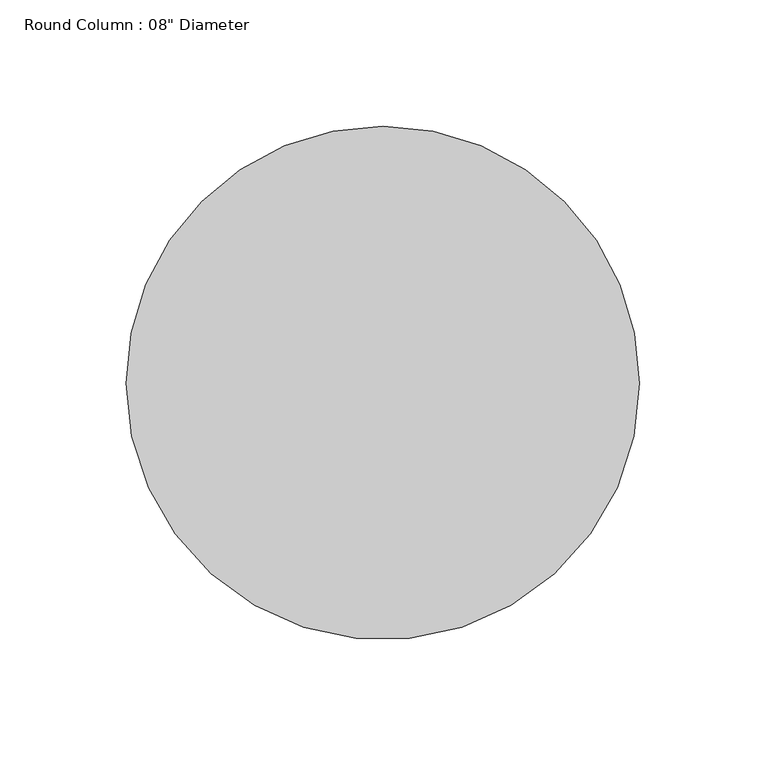
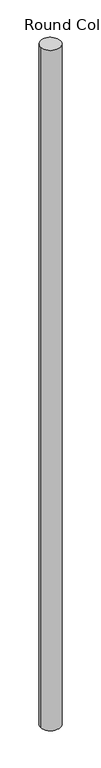
"""IFC4 building model written with IfcOpenShell, lengths in millimetres: column geometry."""

import ifcopenshell
import ifcopenshell.guid

model = None  # the IFC model being written
_history = None  # IfcOwnerHistory: only IFC2X3 demands one
_inside = {}  # id of a spatial element -> (the spatial element, [elements in it])
_under = {}  # id of a project, library or spatial element -> (it, [spatial elements below it])
_declared = {}  # id of a project -> (the project, [libraries it declares])
_typed = {}  # id of a type object -> (the type object, [elements of that type])
_made_of = {}  # id of a material, layer set ... -> (it, [elements and type objects made of it])


def new_model(schema):
    """Start an empty IFC model of exactly this schema.

    Asked for "IFC4X3", IfcOpenShell would pick the latest addendum, in which some entities
    have other attributes; the version numbers below select the first issue.
    IFC2X3 requires an IfcOwnerHistory on every rooted entity: one is made here for all.
    """
    global model, _history
    if schema == "IFC4X3":
        model = ifcopenshell.file(schema_version=(4, 3, 0, 0))
    else:
        model = ifcopenshell.file(schema=schema)
    _inside.clear()
    _under.clear()
    _declared.clear()
    _typed.clear()
    _made_of.clear()
    _history = None
    if model.schema == "IFC2X3":
        org = make("IfcOrganization", Name="unknown")
        user = make(
            "IfcPersonAndOrganization",
            ThePerson=make("IfcPerson", FamilyName="unknown"),
            TheOrganization=org,
        )
        app = make(
            "IfcApplication",
            ApplicationDeveloper=org,
            Version="unknown",
            ApplicationFullName="unknown",
            ApplicationIdentifier="unknown",
        )
        _history = make(
            "IfcOwnerHistory",
            OwningUser=user,
            OwningApplication=app,
            ChangeAction="ADDED",
            CreationDate=0,
        )
    return model


def make(cls, **values):
    """One entity of the class cls with the attributes given. An attribute that is None is left unset."""
    return model.create_entity(
        cls, **{name: value for name, value in values.items() if value is not None}
    )


def rooted(cls, **values):
    """An entity with a GlobalId (a new one), such as an element, a storey or a relation."""
    return make(cls, GlobalId=ifcopenshell.guid.new(), OwnerHistory=_history, **values)


def si_unit(unit_type, name, prefix=None):
    """IfcSIUnit, for example si_unit("LENGTHUNIT", "METRE", prefix="MILLI")."""
    return make("IfcSIUnit", UnitType=unit_type, Prefix=prefix, Name=name)


def assignment(units):
    """IfcUnitAssignment: the units of a project."""
    return None if units is None else make("IfcUnitAssignment", Units=units)


def point(xyz):
    """IfcCartesianPoint."""
    return None if xyz is None else make("IfcCartesianPoint", Coordinates=xyz)


def direction(xyz):
    """IfcDirection."""
    return None if xyz is None else make("IfcDirection", DirectionRatios=xyz)


def frame(location, z_axis=None, x_axis=None):
    """IfcAxis2Placement3D, a coordinate frame: its origin and axes. An axis left out is left unset."""
    return make(
        "IfcAxis2Placement3D",
        Location=point(location),
        Axis=direction(z_axis),
        RefDirection=direction(x_axis),
    )


def frame_2d(location, x_axis=None):
    """IfcAxis2Placement2D, a coordinate frame in the plane: its origin and x axis."""
    return make(
        "IfcAxis2Placement2D", Location=point(location), RefDirection=direction(x_axis)
    )


def origin():
    """The frame at (0, 0, 0) with its axes left unset."""
    return frame((0.0, 0.0, 0.0))


def origin_with_axes():
    """The frame at (0, 0, 0) with the z axis (0, 0, 1) and the x axis (1, 0, 0) written out."""
    return frame((0.0, 0.0, 0.0), z_axis=(0.0, 0.0, 1.0), x_axis=(1.0, 0.0, 0.0))


def origin_2d():
    """The frame at (0, 0) in the plane with its x axis left unset."""
    return frame_2d((0.0, 0.0))


def place(relative_to, where):
    """IfcLocalPlacement: puts the frame where relative to a parent placement (None: the world)."""
    return make(
        "IfcLocalPlacement", PlacementRelTo=relative_to, RelativePlacement=where
    )


def context(
    kind, dimensions, precision=None, world=None, true_north=None, identifier=None
):
    """IfcGeometricRepresentationContext, for example the 3D "Model" context."""
    return make(
        "IfcGeometricRepresentationContext",
        ContextIdentifier=identifier,
        ContextType=kind,
        CoordinateSpaceDimension=dimensions,
        Precision=precision,
        WorldCoordinateSystem=world,
        TrueNorth=true_north,
    )


def project(units=None, contexts=None):
    """IfcProject with its units and contexts."""
    return rooted(
        "IfcProject",
        Name="project",
        RepresentationContexts=contexts,
        UnitsInContext=assignment(units),
    )


def spatial(cls, under=None, at=None, **own):
    """A site, building, storey or space (cls), placed at a placement, below another one or the project."""
    s = rooted(cls, ObjectPlacement=at, **own)
    if under is not None:
        _under.setdefault(under.id(), (under, []))[1].append(s)
    return s


def circle_curve(where, radius):
    """IfcCircle in the frame where."""
    return make("IfcCircle", Position=where, Radius=radius)


def trimmed(basis, trim1, trim2, sense, master):
    """IfcTrimmedCurve: the piece of a basis curve between two trims."""
    return make(
        "IfcTrimmedCurve",
        BasisCurve=basis,
        Trim1=trim1,
        Trim2=trim2,
        SenseAgreement=sense,
        MasterRepresentation=master,
    )


def segment(curve, same_sense, transition):
    """IfcCompositeCurveSegment."""
    return make(
        "IfcCompositeCurveSegment",
        Transition=transition,
        SameSense=same_sense,
        ParentCurve=curve,
    )


def composite_curve(segments, self_intersect=None):
    """IfcCompositeCurve: segments joined end to end."""
    return make("IfcCompositeCurve", Segments=segments, SelfIntersect=self_intersect)


def outline(outer, holes=None, kind="AREA"):
    """IfcArbitraryClosedProfileDef: a profile drawn as a closed curve; with holes, ...WithVoids."""
    if holes is None:
        return make("IfcArbitraryClosedProfileDef", ProfileType=kind, OuterCurve=outer)
    return make(
        "IfcArbitraryProfileDefWithVoids",
        ProfileType=kind,
        OuterCurve=outer,
        InnerCurves=holes,
    )


def extrude(swept, where, along, depth):
    """IfcExtrudedAreaSolid: the profile swept, set in the frame where, extruded along a direction by depth."""
    return make(
        "IfcExtrudedAreaSolid",
        SweptArea=swept,
        Position=where,
        ExtrudedDirection=direction(along),
        Depth=depth,
    )


def shape(context_of_items, identifier, shape_type, items):
    """IfcShapeRepresentation: the items that make up one representation, for example the "Body"."""
    return make(
        "IfcShapeRepresentation",
        ContextOfItems=context_of_items,
        RepresentationIdentifier=identifier,
        RepresentationType=shape_type,
        Items=items,
    )


def source(mapping_origin, context_of_items, identifier, shape_type, items):
    """IfcRepresentationMap: a shape defined once, which mapped items show again and again."""
    return make(
        "IfcRepresentationMap",
        MappingOrigin=mapping_origin,
        MappedRepresentation=shape(context_of_items, identifier, shape_type, items),
    )


def transform(
    local_origin,
    x_axis=None,
    y_axis=None,
    z_axis=None,
    scale=None,
    scale2=None,
    scale3=None,
    uniform=True,
):
    """IfcCartesianTransformationOperator3D, or its non-uniform kind. x_axis, y_axis, z_axis: its Axis1, 2, 3."""
    if uniform:
        return make(
            "IfcCartesianTransformationOperator3D",
            Axis1=direction(x_axis),
            Axis2=direction(y_axis),
            LocalOrigin=point(local_origin),
            Scale=scale,
            Axis3=direction(z_axis),
        )
    return make(
        "IfcCartesianTransformationOperator3DnonUniform",
        Axis1=direction(x_axis),
        Axis2=direction(y_axis),
        LocalOrigin=point(local_origin),
        Scale=scale,
        Axis3=direction(z_axis),
        Scale2=scale2,
        Scale3=scale3,
    )


def mapped(mapping_source, mapping_target):
    """IfcMappedItem: shows the shape of a source again, moved by a transform."""
    return make(
        "IfcMappedItem", MappingSource=mapping_source, MappingTarget=mapping_target
    )


def made_of(thing, what):
    """Note that an element or type object is made of a material, layer set ...; save() writes the relation."""
    if what is not None:
        _made_of.setdefault(what.id(), (what, []))[1].append(thing)
    return thing


def element(
    cls,
    number,
    at=None,
    inside=None,
    cuts=None,
    type_object=None,
    material=None,
    context=None,
    identifier="Body",
    shape_type=None,
    held_by="IfcProductDefinitionShape",
    body=None,
    shapes=None,
    **own,
):
    """One element of the class cls, such as IfcWall. Its Tag is "e" and its number.

    at: its placement. inside: the storey or other place that contains it. cuts: it is an
    opening in that element (IfcRelVoidsElement). A single representation is given by context,
    identifier, shape_type and body (its items); several are given by shapes. held_by: the class
    of the entity that holds the representations. save() writes the other relations.
    """
    e = rooted(cls, Tag="e%d" % number, ObjectPlacement=at, **own)
    if body is not None:
        shapes = [shape(context, identifier, shape_type, body)]
    if shapes is not None:
        e.Representation = make(held_by, Representations=shapes)
    if inside is not None:
        _inside.setdefault(inside.id(), (inside, []))[1].append(e)
    if cuts is not None:
        rooted(
            "IfcRelVoidsElement", RelatingBuildingElement=cuts, RelatedOpeningElement=e
        )
    if type_object is not None:
        _typed.setdefault(type_object.id(), (type_object, []))[1].append(e)
    return made_of(e, material)


def aggregate(whole, parts):
    """IfcRelAggregates: a whole, such as a stair, and the parts it consists of."""
    return rooted("IfcRelAggregates", RelatingObject=whole, RelatedObjects=parts)


def save(model, path):
    """Write the relations noted so far, then the file.

    IfcRelAggregates (storeys below a building ...), IfcRelContainedInSpatialStructure (elements
    in a storey), IfcRelDefinesByType, IfcRelAssociatesMaterial and IfcRelDeclares: one each for
    every whole, place, type object, material and project.
    """
    for whole, parts in _under.values():
        aggregate(whole, parts)
    for where, things in _inside.values():
        rooted(
            "IfcRelContainedInSpatialStructure",
            RelatedElements=things,
            RelatingStructure=where,
        )
    for kind, things in _typed.values():
        rooted("IfcRelDefinesByType", RelatedObjects=things, RelatingType=kind)
    for what, things in _made_of.values():
        rooted("IfcRelAssociatesMaterial", RelatedObjects=things, RelatingMaterial=what)
    for by, libraries in _declared.values():
        rooted("IfcRelDeclares", RelatingContext=by, RelatedDefinitions=libraries)
    model.write(path)


def column_ba67bdda(model_context):
    return source(origin(), model_context, "Body", "SweptSolid", [
        extrude(outline(composite_curve([segment(trimmed(circle_curve(origin_2d(), 101.6), [point((101.6, 0.0))], [point((-101.6, 0.0))], False, "CARTESIAN"), True, "CONTINUOUS"), segment(trimmed(circle_curve(origin_2d(), 101.6), [point((-101.6, 0.0))], [point((0.0, 101.6))], False, "CARTESIAN"), True, "CONTINUOUS"), segment(trimmed(circle_curve(origin_2d(), 101.6), [point((0.0, 101.6))], [point((101.6, 0.0))], False, "CARTESIAN"), True, "CONTINUOUS")], self_intersect=False)), origin_with_axes(), (0.0, 0.0, 1.0), 7315.2),
    ])


if __name__ == "__main__":
    model = new_model("IFC4")
    model_context = context("Model", 3, world=origin())
    ifc_project = project(units=[si_unit("LENGTHUNIT", "METRE", prefix="MILLI")], contexts=[model_context])
    site = spatial("IfcSite", under=ifc_project)
    building = spatial("IfcBuilding", under=site)
    placement = place(None, origin())
    column_shape = column_ba67bdda(model_context)
    element("IfcColumn", 1, ObjectType="Round Column : 08\" Diameter", at=placement, inside=building, context=model_context, shape_type="MappedRepresentation", body=[
        mapped(column_shape, transform((0.0, 0.0, 0.0), x_axis=(1.0, 0.0, 0.0), y_axis=(0.0, 1.0, 0.0), z_axis=(0.0, 0.0, 1.0))),
    ])
    save(model, "model.ifc")

# Revit data of these elements
# Type "Round Column : 08\" Diameter"
#   Assembly Code = "B1010200"
#   Diameter = 203.20 mm
#   Offset Base = 0.00 mm
#   Offset Top = 0.00 mm
#   Material = none
